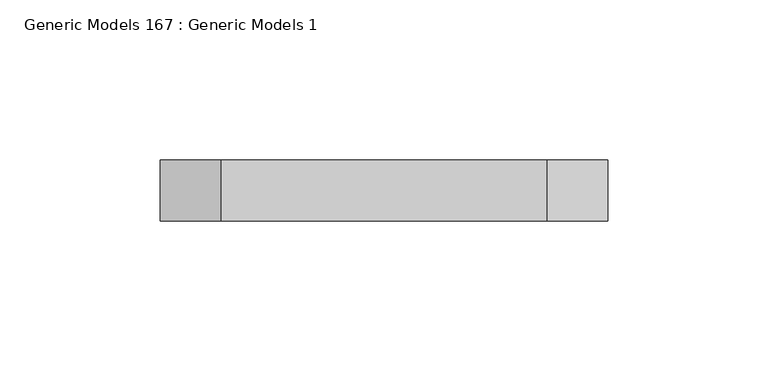
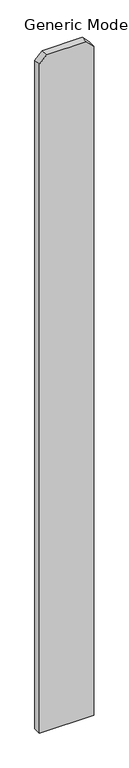
"""IFC4 building model written with IfcOpenShell, lengths in millimetres: proxy geometry, Generic Models 167 : Generic Models 1."""

from ifc_helpers import new_model, si_unit, frame, origin, place, context, project, spatial, polyline, outline, extrude, source, transform, mapped, element, save


def generic_models_167_generic_models_1_e84e9edf(model_context):
    return source(origin(), model_context, "Body", "SweptSolid", [
        extrude(outline(polyline([(76.2, -249353.3875), (1885.95, -249353.3875), (1905.0, -249372.4375), (1905.0, -249474.0375), (1885.95, -249493.0875), (76.2, -249493.0875), (76.2, -249353.3875)])), frame((0.0, 547.6875, 0.0), z_axis=(0.0, 1.0, 0.0), x_axis=(0.0, 0.0, 1.0)), (0.0, 0.0, 1.0), 19.05),
    ])


if __name__ == "__main__":
    model = new_model("IFC4")
    model_context = context("Model", 3, world=origin())
    ifc_project = project(units=[si_unit("LENGTHUNIT", "METRE", prefix="MILLI")], contexts=[model_context])
    site = spatial("IfcSite", under=ifc_project)
    building = spatial("IfcBuilding", under=site)
    placement = place(None, origin())
    generic_models_167_generic_models_1_shape = generic_models_167_generic_models_1_e84e9edf(model_context)
    element("IfcBuildingElementProxy", 1, Name="Generic Models 167 : Generic Models 1", ObjectType="Generic Models 167 : Generic Models 1", at=placement, inside=building, context=model_context, shape_type="MappedRepresentation", body=[
        mapped(generic_models_167_generic_models_1_shape, transform((0.0, 0.0, 0.0), x_axis=(1.0, 0.0, 0.0), y_axis=(0.0, 1.0, 0.0), z_axis=(0.0, 0.0, 1.0))),
    ])
    save(model, "model.ifc")

# Revit data of these elements
# Element 1 (IfcBuildingElementProxy, "Generic Models 167 : Generic Models 1")
#   Materials on its faces: "VERTICAL 1X6 CEDAR PLANKS W/ CLEAR WOOD SEALER"
# Materials
#   "VERTICAL 1X6 CEDAR PLANKS W/ CLEAR WOOD SEALER": class "Wood", colour RGB 234 198 147, transparency 0, Description = "Pinus Echinata", Cost = 0
